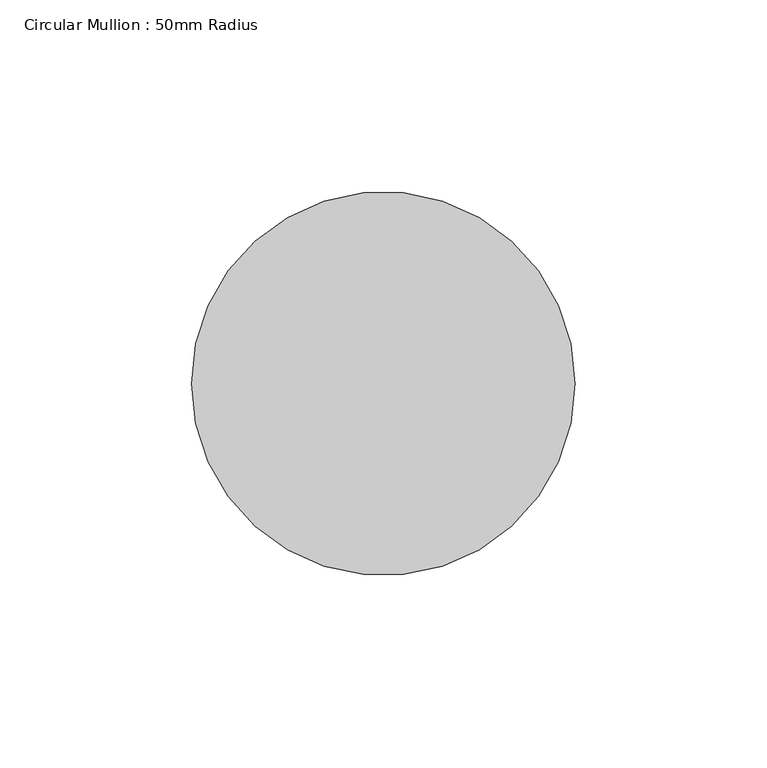
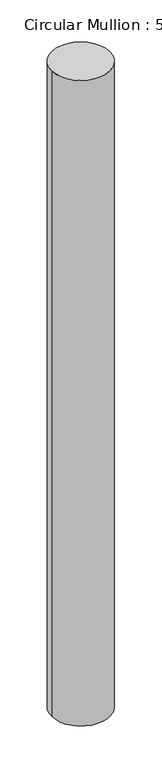
"""IFC4 building model written with IfcOpenShell, lengths in millimetres: member geometry, Circular Mullion : 50mm Radius."""

from ifc_helpers import new_model, si_unit, point, frame, origin, origin_2d, place, context, project, spatial, circle_curve, trimmed, segment, composite_curve, outline, extrude, source, transform, mapped, element, save


def circular_mullion_50mm_radius_47b50501(model_context):
    return source(origin(), model_context, "Body", "SweptSolid", [
        extrude(outline(composite_curve([segment(trimmed(circle_curve(origin_2d(), 50.0), [point((50.0, 0.0))], [point((-50.0, 0.0))], False, "CARTESIAN"), True, "CONTINUOUS"), segment(trimmed(circle_curve(origin_2d(), 50.0), [point((-50.0, 0.0))], [point((50.0, 0.0))], False, "CARTESIAN"), True, "CONTINUOUS")], self_intersect=False)), frame((0.0, 0.0, -1173.8989178), z_axis=(0.0, 0.0, 1.0), x_axis=(1.0, 0.0, 0.0)), (0.0, 0.0, 1.0), 1173.8989178),
    ])


if __name__ == "__main__":
    model = new_model("IFC4")
    model_context = context("Model", 3, world=origin())
    ifc_project = project(units=[si_unit("LENGTHUNIT", "METRE", prefix="MILLI")], contexts=[model_context])
    site = spatial("IfcSite", under=ifc_project)
    building = spatial("IfcBuilding", under=site)
    placement = place(None, origin())
    circular_mullion_50mm_radius_shape = circular_mullion_50mm_radius_47b50501(model_context)
    element("IfcMember", 1, ObjectType="Circular Mullion : 50mm Radius", at=placement, inside=building, context=model_context, shape_type="MappedRepresentation", body=[
        mapped(circular_mullion_50mm_radius_shape, transform((0.0, 0.0, 0.0), x_axis=(1.0, 0.0, 0.0), y_axis=(0.0, 1.0, 0.0), z_axis=(0.0, 0.0, 1.0))),
    ])
    save(model, "model.ifc")

# Revit data of these elements
# Type "Circular Mullion : 50mm Radius"
#   built-in parameter 1007350 = 0.164042 (stored number, unit not read)
# Element 1 (IfcMember, "Circular Mullion : 50mm Radius")
#   Materials on its faces: "Aluminium"
# Materials
#   "Aluminium": class "Metal", colour RGB 247 247 247, transparency 0, Description = "Aluminium 6061", Cost = 0
